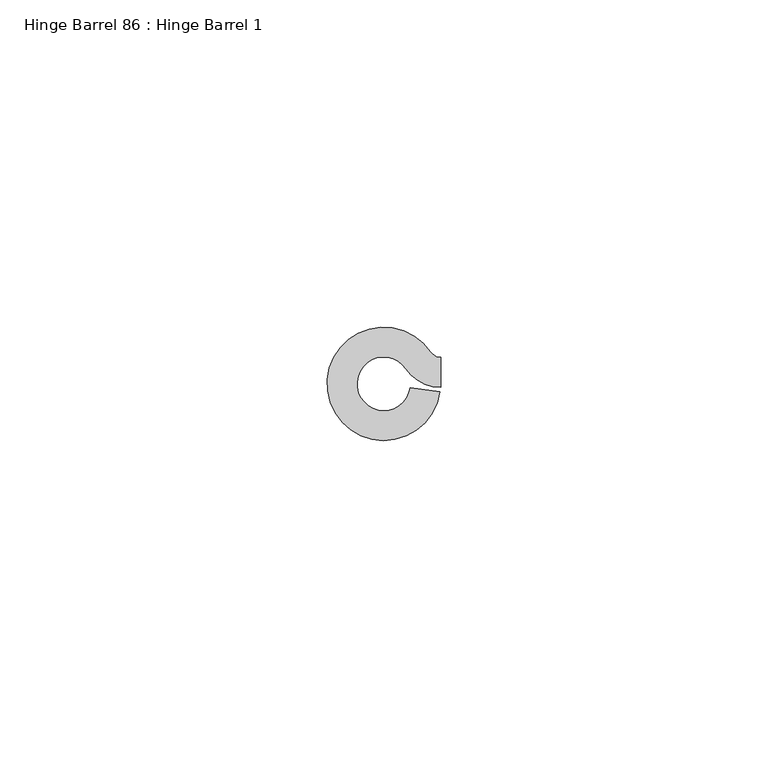
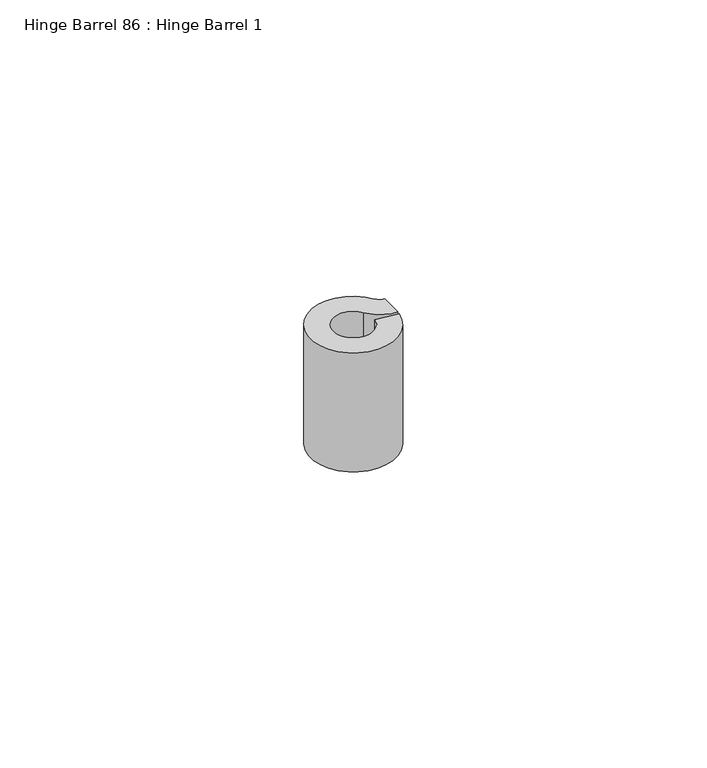
"""IFC4 building model written with IfcOpenShell, lengths in millimetres: proxy geometry, Hinge Barrel 86 : Hinge Barrel 1."""

import ifcopenshell
import ifcopenshell.guid

model = None  # the IFC model being written
_history = None  # IfcOwnerHistory: only IFC2X3 demands one
_inside = {}  # id of a spatial element -> (the spatial element, [elements in it])
_under = {}  # id of a project, library or spatial element -> (it, [spatial elements below it])
_declared = {}  # id of a project -> (the project, [libraries it declares])
_typed = {}  # id of a type object -> (the type object, [elements of that type])
_made_of = {}  # id of a material, layer set ... -> (it, [elements and type objects made of it])


def new_model(schema):
    """Start an empty IFC model of exactly this schema.

    Asked for "IFC4X3", IfcOpenShell would pick the latest addendum, in which some entities
    have other attributes; the version numbers below select the first issue.
    IFC2X3 requires an IfcOwnerHistory on every rooted entity: one is made here for all.
    """
    global model, _history
    if schema == "IFC4X3":
        model = ifcopenshell.file(schema_version=(4, 3, 0, 0))
    else:
        model = ifcopenshell.file(schema=schema)
    _inside.clear()
    _under.clear()
    _declared.clear()
    _typed.clear()
    _made_of.clear()
    _history = None
    if model.schema == "IFC2X3":
        org = make("IfcOrganization", Name="unknown")
        user = make(
            "IfcPersonAndOrganization",
            ThePerson=make("IfcPerson", FamilyName="unknown"),
            TheOrganization=org,
        )
        app = make(
            "IfcApplication",
            ApplicationDeveloper=org,
            Version="unknown",
            ApplicationFullName="unknown",
            ApplicationIdentifier="unknown",
        )
        _history = make(
            "IfcOwnerHistory",
            OwningUser=user,
            OwningApplication=app,
            ChangeAction="ADDED",
            CreationDate=0,
        )
    return model


def make(cls, **values):
    """One entity of the class cls with the attributes given. An attribute that is None is left unset."""
    return model.create_entity(
        cls, **{name: value for name, value in values.items() if value is not None}
    )


def rooted(cls, **values):
    """An entity with a GlobalId (a new one), such as an element, a storey or a relation."""
    return make(cls, GlobalId=ifcopenshell.guid.new(), OwnerHistory=_history, **values)


def si_unit(unit_type, name, prefix=None):
    """IfcSIUnit, for example si_unit("LENGTHUNIT", "METRE", prefix="MILLI")."""
    return make("IfcSIUnit", UnitType=unit_type, Prefix=prefix, Name=name)


def assignment(units):
    """IfcUnitAssignment: the units of a project."""
    return None if units is None else make("IfcUnitAssignment", Units=units)


def point(xyz):
    """IfcCartesianPoint."""
    return None if xyz is None else make("IfcCartesianPoint", Coordinates=xyz)


def direction(xyz):
    """IfcDirection."""
    return None if xyz is None else make("IfcDirection", DirectionRatios=xyz)


def frame(location, z_axis=None, x_axis=None):
    """IfcAxis2Placement3D, a coordinate frame: its origin and axes. An axis left out is left unset."""
    return make(
        "IfcAxis2Placement3D",
        Location=point(location),
        Axis=direction(z_axis),
        RefDirection=direction(x_axis),
    )


def frame_2d(location, x_axis=None):
    """IfcAxis2Placement2D, a coordinate frame in the plane: its origin and x axis."""
    return make(
        "IfcAxis2Placement2D", Location=point(location), RefDirection=direction(x_axis)
    )


def origin():
    """The frame at (0, 0, 0) with its axes left unset."""
    return frame((0.0, 0.0, 0.0))


def place(relative_to, where):
    """IfcLocalPlacement: puts the frame where relative to a parent placement (None: the world)."""
    return make(
        "IfcLocalPlacement", PlacementRelTo=relative_to, RelativePlacement=where
    )


def context(
    kind, dimensions, precision=None, world=None, true_north=None, identifier=None
):
    """IfcGeometricRepresentationContext, for example the 3D "Model" context."""
    return make(
        "IfcGeometricRepresentationContext",
        ContextIdentifier=identifier,
        ContextType=kind,
        CoordinateSpaceDimension=dimensions,
        Precision=precision,
        WorldCoordinateSystem=world,
        TrueNorth=true_north,
    )


def project(units=None, contexts=None):
    """IfcProject with its units and contexts."""
    return rooted(
        "IfcProject",
        Name="project",
        RepresentationContexts=contexts,
        UnitsInContext=assignment(units),
    )


def spatial(cls, under=None, at=None, **own):
    """A site, building, storey or space (cls), placed at a placement, below another one or the project."""
    s = rooted(cls, ObjectPlacement=at, **own)
    if under is not None:
        _under.setdefault(under.id(), (under, []))[1].append(s)
    return s


def polyline(points):
    """IfcPolyline through the points."""
    return make("IfcPolyline", Points=[point(p) for p in points])


def circle_curve(where, radius):
    """IfcCircle in the frame where."""
    return make("IfcCircle", Position=where, Radius=radius)


def trimmed(basis, trim1, trim2, sense, master):
    """IfcTrimmedCurve: the piece of a basis curve between two trims."""
    return make(
        "IfcTrimmedCurve",
        BasisCurve=basis,
        Trim1=trim1,
        Trim2=trim2,
        SenseAgreement=sense,
        MasterRepresentation=master,
    )


def segment(curve, same_sense, transition):
    """IfcCompositeCurveSegment."""
    return make(
        "IfcCompositeCurveSegment",
        Transition=transition,
        SameSense=same_sense,
        ParentCurve=curve,
    )


def composite_curve(segments, self_intersect=None):
    """IfcCompositeCurve: segments joined end to end."""
    return make("IfcCompositeCurve", Segments=segments, SelfIntersect=self_intersect)


def outline(outer, holes=None, kind="AREA"):
    """IfcArbitraryClosedProfileDef: a profile drawn as a closed curve; with holes, ...WithVoids."""
    if holes is None:
        return make("IfcArbitraryClosedProfileDef", ProfileType=kind, OuterCurve=outer)
    return make(
        "IfcArbitraryProfileDefWithVoids",
        ProfileType=kind,
        OuterCurve=outer,
        InnerCurves=holes,
    )


def extrude(swept, where, along, depth):
    """IfcExtrudedAreaSolid: the profile swept, set in the frame where, extruded along a direction by depth."""
    return make(
        "IfcExtrudedAreaSolid",
        SweptArea=swept,
        Position=where,
        ExtrudedDirection=direction(along),
        Depth=depth,
    )


def shape(context_of_items, identifier, shape_type, items):
    """IfcShapeRepresentation: the items that make up one representation, for example the "Body"."""
    return make(
        "IfcShapeRepresentation",
        ContextOfItems=context_of_items,
        RepresentationIdentifier=identifier,
        RepresentationType=shape_type,
        Items=items,
    )


def source(mapping_origin, context_of_items, identifier, shape_type, items):
    """IfcRepresentationMap: a shape defined once, which mapped items show again and again."""
    return make(
        "IfcRepresentationMap",
        MappingOrigin=mapping_origin,
        MappedRepresentation=shape(context_of_items, identifier, shape_type, items),
    )


def transform(
    local_origin,
    x_axis=None,
    y_axis=None,
    z_axis=None,
    scale=None,
    scale2=None,
    scale3=None,
    uniform=True,
):
    """IfcCartesianTransformationOperator3D, or its non-uniform kind. x_axis, y_axis, z_axis: its Axis1, 2, 3."""
    if uniform:
        return make(
            "IfcCartesianTransformationOperator3D",
            Axis1=direction(x_axis),
            Axis2=direction(y_axis),
            LocalOrigin=point(local_origin),
            Scale=scale,
            Axis3=direction(z_axis),
        )
    return make(
        "IfcCartesianTransformationOperator3DnonUniform",
        Axis1=direction(x_axis),
        Axis2=direction(y_axis),
        LocalOrigin=point(local_origin),
        Scale=scale,
        Axis3=direction(z_axis),
        Scale2=scale2,
        Scale3=scale3,
    )


def mapped(mapping_source, mapping_target):
    """IfcMappedItem: shows the shape of a source again, moved by a transform."""
    return make(
        "IfcMappedItem", MappingSource=mapping_source, MappingTarget=mapping_target
    )


def made_of(thing, what):
    """Note that an element or type object is made of a material, layer set ...; save() writes the relation."""
    if what is not None:
        _made_of.setdefault(what.id(), (what, []))[1].append(thing)
    return thing


def element(
    cls,
    number,
    at=None,
    inside=None,
    cuts=None,
    type_object=None,
    material=None,
    context=None,
    identifier="Body",
    shape_type=None,
    held_by="IfcProductDefinitionShape",
    body=None,
    shapes=None,
    **own,
):
    """One element of the class cls, such as IfcWall. Its Tag is "e" and its number.

    at: its placement. inside: the storey or other place that contains it. cuts: it is an
    opening in that element (IfcRelVoidsElement). A single representation is given by context,
    identifier, shape_type and body (its items); several are given by shapes. held_by: the class
    of the entity that holds the representations. save() writes the other relations.
    """
    e = rooted(cls, Tag="e%d" % number, ObjectPlacement=at, **own)
    if body is not None:
        shapes = [shape(context, identifier, shape_type, body)]
    if shapes is not None:
        e.Representation = make(held_by, Representations=shapes)
    if inside is not None:
        _inside.setdefault(inside.id(), (inside, []))[1].append(e)
    if cuts is not None:
        rooted(
            "IfcRelVoidsElement", RelatingBuildingElement=cuts, RelatedOpeningElement=e
        )
    if type_object is not None:
        _typed.setdefault(type_object.id(), (type_object, []))[1].append(e)
    return made_of(e, material)


def aggregate(whole, parts):
    """IfcRelAggregates: a whole, such as a stair, and the parts it consists of."""
    return rooted("IfcRelAggregates", RelatingObject=whole, RelatedObjects=parts)


def save(model, path):
    """Write the relations noted so far, then the file.

    IfcRelAggregates (storeys below a building ...), IfcRelContainedInSpatialStructure (elements
    in a storey), IfcRelDefinesByType, IfcRelAssociatesMaterial and IfcRelDeclares: one each for
    every whole, place, type object, material and project.
    """
    for whole, parts in _under.values():
        aggregate(whole, parts)
    for where, things in _inside.values():
        rooted(
            "IfcRelContainedInSpatialStructure",
            RelatedElements=things,
            RelatingStructure=where,
        )
    for kind, things in _typed.values():
        rooted("IfcRelDefinesByType", RelatedObjects=things, RelatingType=kind)
    for what, things in _made_of.values():
        rooted("IfcRelAssociatesMaterial", RelatedObjects=things, RelatingMaterial=what)
    for by, libraries in _declared.values():
        rooted("IfcRelDeclares", RelatingContext=by, RelatedDefinitions=libraries)
    model.write(path)


def hinge_barrel_86_hinge_barrel_1_b61994a4(model_context):
    return source(origin(), model_context, "Body", "SweptSolid", [
        extrude(outline(composite_curve([segment(trimmed(circle_curve(frame_2d((587319.1320739, -531776.6049841)), 4.0894), [point((587322.5194669, -531774.3139665))], [point((587323.1821338, -531777.1708529))], True, "CARTESIAN"), True, "CONTINUOUS"), segment(polyline([(587323.1821338, -531777.1708529), (587327.7022899, -531777.8024028)]), True, "CONTINUOUS"), segment(trimmed(circle_curve(frame_2d((587319.1320739, -531776.6049841)), 8.6534625), [point((587327.7022899, -531777.8024028))], [point((587326.3000393, -531771.7570273))], False, "CARTESIAN"), True, "CONTINUOUS"), segment(trimmed(circle_curve(frame_2d((587327.8245257, -531770.7259615)), 1.8404226), [point((587326.3000393, -531771.7570273))], [point((587327.8245257, -531772.5663841))], True, "CARTESIAN"), True, "CONTINUOUS"), segment(polyline([(587327.8245257, -531772.5663841), (587327.8245257, -531777.1304466)]), True, "CONTINUOUS"), segment(trimmed(circle_curve(frame_2d((587327.8245257, -531770.7259615)), 6.4044851), [point((587327.8245257, -531777.1304466))], [point((587322.5194669, -531774.3139665))], False, "CARTESIAN"), True, "CONTINUOUS")], self_intersect=False)), frame((0.0, 0.0, 1149.35), z_axis=(0.0, 0.0, 1.0), x_axis=(1.0, 0.0, 0.0)), (0.0, 0.0, 1.0), 25.4),
    ])


if __name__ == "__main__":
    model = new_model("IFC4")
    model_context = context("Model", 3, world=origin())
    ifc_project = project(units=[si_unit("LENGTHUNIT", "METRE", prefix="MILLI")], contexts=[model_context])
    site = spatial("IfcSite", under=ifc_project)
    building = spatial("IfcBuilding", under=site)
    placement = place(None, origin())
    hinge_barrel_86_hinge_barrel_1_shape = hinge_barrel_86_hinge_barrel_1_b61994a4(model_context)
    element("IfcBuildingElementProxy", 1, Name="Hinge Barrel 86 : Hinge Barrel 1", ObjectType="Hinge Barrel 86 : Hinge Barrel 1", at=placement, inside=building, context=model_context, shape_type="MappedRepresentation", body=[
        mapped(hinge_barrel_86_hinge_barrel_1_shape, transform((0.0, 0.0, 0.0), x_axis=(1.0, 0.0, 0.0), y_axis=(0.0, 1.0, 0.0), z_axis=(0.0, 0.0, 1.0))),
    ])
    save(model, "model.ifc")

# Revit data of these elements
# Element 1 (IfcBuildingElementProxy, "Hinge Barrel 86 : Hinge Barrel 1")
#   Materials on its faces: "6\"X6\" WELD-ON STL BUTT HINGE"
# Materials
#   "6\"X6\" WELD-ON STL BUTT HINGE": class "Metal", colour RGB 189 187 185, transparency 0, Description = "Carbon steel", Cost = 0
